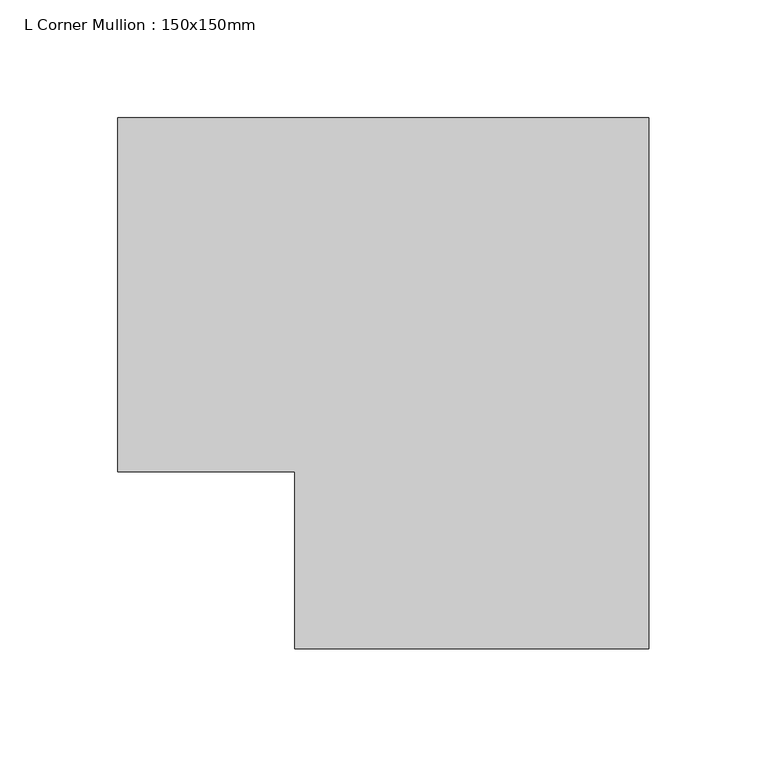
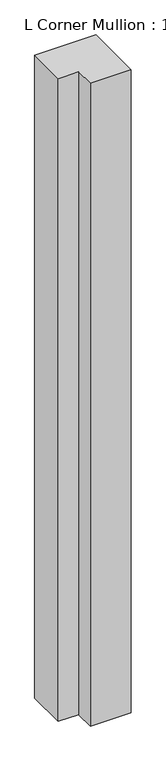
"""IFC4 building model written with IfcOpenShell, lengths in millimetres: member geometry, L Corner Mullion : 150x150mm."""

import ifcopenshell
import ifcopenshell.guid

model = None  # the IFC model being written
_history = None  # IfcOwnerHistory: only IFC2X3 demands one
_inside = {}  # id of a spatial element -> (the spatial element, [elements in it])
_under = {}  # id of a project, library or spatial element -> (it, [spatial elements below it])
_declared = {}  # id of a project -> (the project, [libraries it declares])
_typed = {}  # id of a type object -> (the type object, [elements of that type])
_made_of = {}  # id of a material, layer set ... -> (it, [elements and type objects made of it])


def new_model(schema):
    """Start an empty IFC model of exactly this schema.

    Asked for "IFC4X3", IfcOpenShell would pick the latest addendum, in which some entities
    have other attributes; the version numbers below select the first issue.
    IFC2X3 requires an IfcOwnerHistory on every rooted entity: one is made here for all.
    """
    global model, _history
    if schema == "IFC4X3":
        model = ifcopenshell.file(schema_version=(4, 3, 0, 0))
    else:
        model = ifcopenshell.file(schema=schema)
    _inside.clear()
    _under.clear()
    _declared.clear()
    _typed.clear()
    _made_of.clear()
    _history = None
    if model.schema == "IFC2X3":
        org = make("IfcOrganization", Name="unknown")
        user = make(
            "IfcPersonAndOrganization",
            ThePerson=make("IfcPerson", FamilyName="unknown"),
            TheOrganization=org,
        )
        app = make(
            "IfcApplication",
            ApplicationDeveloper=org,
            Version="unknown",
            ApplicationFullName="unknown",
            ApplicationIdentifier="unknown",
        )
        _history = make(
            "IfcOwnerHistory",
            OwningUser=user,
            OwningApplication=app,
            ChangeAction="ADDED",
            CreationDate=0,
        )
    return model


def make(cls, **values):
    """One entity of the class cls with the attributes given. An attribute that is None is left unset."""
    return model.create_entity(
        cls, **{name: value for name, value in values.items() if value is not None}
    )


def rooted(cls, **values):
    """An entity with a GlobalId (a new one), such as an element, a storey or a relation."""
    return make(cls, GlobalId=ifcopenshell.guid.new(), OwnerHistory=_history, **values)


def si_unit(unit_type, name, prefix=None):
    """IfcSIUnit, for example si_unit("LENGTHUNIT", "METRE", prefix="MILLI")."""
    return make("IfcSIUnit", UnitType=unit_type, Prefix=prefix, Name=name)


def assignment(units):
    """IfcUnitAssignment: the units of a project."""
    return None if units is None else make("IfcUnitAssignment", Units=units)


def point(xyz):
    """IfcCartesianPoint."""
    return None if xyz is None else make("IfcCartesianPoint", Coordinates=xyz)


def direction(xyz):
    """IfcDirection."""
    return None if xyz is None else make("IfcDirection", DirectionRatios=xyz)


def frame(location, z_axis=None, x_axis=None):
    """IfcAxis2Placement3D, a coordinate frame: its origin and axes. An axis left out is left unset."""
    return make(
        "IfcAxis2Placement3D",
        Location=point(location),
        Axis=direction(z_axis),
        RefDirection=direction(x_axis),
    )


def origin():
    """The frame at (0, 0, 0) with its axes left unset."""
    return frame((0.0, 0.0, 0.0))


def place(relative_to, where):
    """IfcLocalPlacement: puts the frame where relative to a parent placement (None: the world)."""
    return make(
        "IfcLocalPlacement", PlacementRelTo=relative_to, RelativePlacement=where
    )


def context(
    kind, dimensions, precision=None, world=None, true_north=None, identifier=None
):
    """IfcGeometricRepresentationContext, for example the 3D "Model" context."""
    return make(
        "IfcGeometricRepresentationContext",
        ContextIdentifier=identifier,
        ContextType=kind,
        CoordinateSpaceDimension=dimensions,
        Precision=precision,
        WorldCoordinateSystem=world,
        TrueNorth=true_north,
    )


def project(units=None, contexts=None):
    """IfcProject with its units and contexts."""
    return rooted(
        "IfcProject",
        Name="project",
        RepresentationContexts=contexts,
        UnitsInContext=assignment(units),
    )


def spatial(cls, under=None, at=None, **own):
    """A site, building, storey or space (cls), placed at a placement, below another one or the project."""
    s = rooted(cls, ObjectPlacement=at, **own)
    if under is not None:
        _under.setdefault(under.id(), (under, []))[1].append(s)
    return s


def polyline(points):
    """IfcPolyline through the points."""
    return make("IfcPolyline", Points=[point(p) for p in points])


def outline(outer, holes=None, kind="AREA"):
    """IfcArbitraryClosedProfileDef: a profile drawn as a closed curve; with holes, ...WithVoids."""
    if holes is None:
        return make("IfcArbitraryClosedProfileDef", ProfileType=kind, OuterCurve=outer)
    return make(
        "IfcArbitraryProfileDefWithVoids",
        ProfileType=kind,
        OuterCurve=outer,
        InnerCurves=holes,
    )


def extrude(swept, where, along, depth):
    """IfcExtrudedAreaSolid: the profile swept, set in the frame where, extruded along a direction by depth."""
    return make(
        "IfcExtrudedAreaSolid",
        SweptArea=swept,
        Position=where,
        ExtrudedDirection=direction(along),
        Depth=depth,
    )


def shape(context_of_items, identifier, shape_type, items):
    """IfcShapeRepresentation: the items that make up one representation, for example the "Body"."""
    return make(
        "IfcShapeRepresentation",
        ContextOfItems=context_of_items,
        RepresentationIdentifier=identifier,
        RepresentationType=shape_type,
        Items=items,
    )


def source(mapping_origin, context_of_items, identifier, shape_type, items):
    """IfcRepresentationMap: a shape defined once, which mapped items show again and again."""
    return make(
        "IfcRepresentationMap",
        MappingOrigin=mapping_origin,
        MappedRepresentation=shape(context_of_items, identifier, shape_type, items),
    )


def transform(
    local_origin,
    x_axis=None,
    y_axis=None,
    z_axis=None,
    scale=None,
    scale2=None,
    scale3=None,
    uniform=True,
):
    """IfcCartesianTransformationOperator3D, or its non-uniform kind. x_axis, y_axis, z_axis: its Axis1, 2, 3."""
    if uniform:
        return make(
            "IfcCartesianTransformationOperator3D",
            Axis1=direction(x_axis),
            Axis2=direction(y_axis),
            LocalOrigin=point(local_origin),
            Scale=scale,
            Axis3=direction(z_axis),
        )
    return make(
        "IfcCartesianTransformationOperator3DnonUniform",
        Axis1=direction(x_axis),
        Axis2=direction(y_axis),
        LocalOrigin=point(local_origin),
        Scale=scale,
        Axis3=direction(z_axis),
        Scale2=scale2,
        Scale3=scale3,
    )


def mapped(mapping_source, mapping_target):
    """IfcMappedItem: shows the shape of a source again, moved by a transform."""
    return make(
        "IfcMappedItem", MappingSource=mapping_source, MappingTarget=mapping_target
    )


def made_of(thing, what):
    """Note that an element or type object is made of a material, layer set ...; save() writes the relation."""
    if what is not None:
        _made_of.setdefault(what.id(), (what, []))[1].append(thing)
    return thing


def element(
    cls,
    number,
    at=None,
    inside=None,
    cuts=None,
    type_object=None,
    material=None,
    context=None,
    identifier="Body",
    shape_type=None,
    held_by="IfcProductDefinitionShape",
    body=None,
    shapes=None,
    **own,
):
    """One element of the class cls, such as IfcWall. Its Tag is "e" and its number.

    at: its placement. inside: the storey or other place that contains it. cuts: it is an
    opening in that element (IfcRelVoidsElement). A single representation is given by context,
    identifier, shape_type and body (its items); several are given by shapes. held_by: the class
    of the entity that holds the representations. save() writes the other relations.
    """
    e = rooted(cls, Tag="e%d" % number, ObjectPlacement=at, **own)
    if body is not None:
        shapes = [shape(context, identifier, shape_type, body)]
    if shapes is not None:
        e.Representation = make(held_by, Representations=shapes)
    if inside is not None:
        _inside.setdefault(inside.id(), (inside, []))[1].append(e)
    if cuts is not None:
        rooted(
            "IfcRelVoidsElement", RelatingBuildingElement=cuts, RelatedOpeningElement=e
        )
    if type_object is not None:
        _typed.setdefault(type_object.id(), (type_object, []))[1].append(e)
    return made_of(e, material)


def aggregate(whole, parts):
    """IfcRelAggregates: a whole, such as a stair, and the parts it consists of."""
    return rooted("IfcRelAggregates", RelatingObject=whole, RelatedObjects=parts)


def save(model, path):
    """Write the relations noted so far, then the file.

    IfcRelAggregates (storeys below a building ...), IfcRelContainedInSpatialStructure (elements
    in a storey), IfcRelDefinesByType, IfcRelAssociatesMaterial and IfcRelDeclares: one each for
    every whole, place, type object, material and project.
    """
    for whole, parts in _under.values():
        aggregate(whole, parts)
    for where, things in _inside.values():
        rooted(
            "IfcRelContainedInSpatialStructure",
            RelatedElements=things,
            RelatingStructure=where,
        )
    for kind, things in _typed.values():
        rooted("IfcRelDefinesByType", RelatedObjects=things, RelatingType=kind)
    for what, things in _made_of.values():
        rooted("IfcRelAssociatesMaterial", RelatedObjects=things, RelatingMaterial=what)
    for by, libraries in _declared.values():
        rooted("IfcRelDeclares", RelatingContext=by, RelatedDefinitions=libraries)
    model.write(path)


def l_corner_mullion_150x150mm_fe080c53(model_context):
    return source(origin(), model_context, "Body", "SweptSolid", [
        extrude(outline(polyline([(-75.0, -150.0), (-75.0, -75.0), (-150.0, -75.0), (-150.0, 75.0), (75.0, 75.0), (75.0, -150.0), (-75.0, -150.0)])), frame((0.0, 0.0, -2500.0), z_axis=(0.0, 0.0, 1.0), x_axis=(1.0, 0.0, 0.0)), (0.0, 0.0, 1.0), 2500.0),
    ])


if __name__ == "__main__":
    model = new_model("IFC4")
    model_context = context("Model", 3, world=origin())
    ifc_project = project(units=[si_unit("LENGTHUNIT", "METRE", prefix="MILLI")], contexts=[model_context])
    site = spatial("IfcSite", under=ifc_project)
    building = spatial("IfcBuilding", under=site)
    placement = place(None, origin())
    l_corner_mullion_150x150mm_shape = l_corner_mullion_150x150mm_fe080c53(model_context)
    element("IfcMember", 1, ObjectType="L Corner Mullion : 150x150mm", at=placement, inside=building, context=model_context, shape_type="MappedRepresentation", body=[
        mapped(l_corner_mullion_150x150mm_shape, transform((0.0, 0.0, 0.0), x_axis=(1.0, 0.0, 0.0), y_axis=(0.0, 1.0, 0.0), z_axis=(0.0, 0.0, 1.0))),
    ])
    save(model, "model.ifc")

# Revit data of these elements
# Type "L Corner Mullion : 150x150mm"
#   Keynote = "H11"
#   built-in parameter 1007355 = 0.492126 (stored number, unit not read)
#   built-in parameter 1007354 = 0.492126 (stored number, unit not read)
#   built-in parameter 1007304 = 0.492126 (stored number, unit not read)
# Element 1 (IfcMember, "L Corner Mullion : 150x150mm")
#   Materials on its faces: "Aluminium"
# Materials
#   "Aluminium": class "Metal", colour RGB 247 247 247, transparency 0, Description = "Aluminium 6061", Cost = 0
